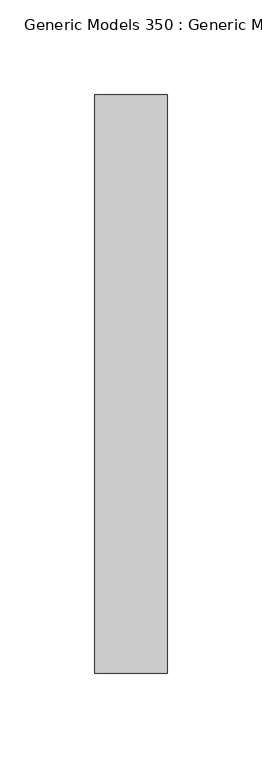
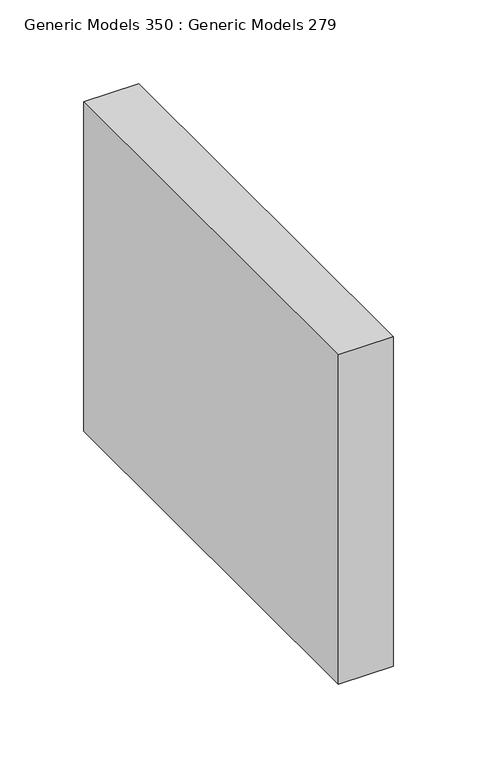
"""IFC4 building model written with IfcOpenShell, lengths in millimetres: proxy geometry, Generic Models 350 : Generic Models 279."""

from ifc_helpers import new_model, si_unit, frame, origin, place, context, project, spatial, polyline, outline, extrude, source, transform, mapped, element, save


def generic_models_350_generic_models_279_699e82a9(model_context):
    return source(origin(), model_context, "Body", "SweptSolid", [
        extrude(outline(polyline([(3531.1804357, 704.5309662), (3569.2804357, 704.5309662), (3569.2804357, 399.7309662), (3531.1804357, 399.7309662), (3531.1804357, 704.5309662)])), frame((0.0, 0.0, 124495.3415398), z_axis=(0.0, 0.0, 1.0), x_axis=(1.0, 0.0, 0.0)), (0.0, 0.0, 1.0), 240.792),
    ])


if __name__ == "__main__":
    model = new_model("IFC4")
    model_context = context("Model", 3, world=origin())
    ifc_project = project(units=[si_unit("LENGTHUNIT", "METRE", prefix="MILLI")], contexts=[model_context])
    site = spatial("IfcSite", under=ifc_project)
    building = spatial("IfcBuilding", under=site)
    placement = place(None, origin())
    generic_models_350_generic_models_279_shape = generic_models_350_generic_models_279_699e82a9(model_context)
    element("IfcBuildingElementProxy", 1, Name="Generic Models 350 : Generic Models 279", ObjectType="Generic Models 350 : Generic Models 279", at=placement, inside=building, context=model_context, shape_type="MappedRepresentation", body=[
        mapped(generic_models_350_generic_models_279_shape, transform((0.0, 0.0, 0.0), x_axis=(1.0, 0.0, 0.0), y_axis=(0.0, 1.0, 0.0), z_axis=(0.0, 0.0, 1.0))),
    ])
    save(model, "model.ifc")

# Revit data of these elements
# Element 1 (IfcBuildingElementProxy, "Generic Models 350 : Generic Models 279")
#   Materials on its faces: "_BLOCKING AS REQUIRED"
# Materials
#   "_BLOCKING AS REQUIRED": class "Generic", colour RGB 177 130 114, transparency 0, Cost = 0
